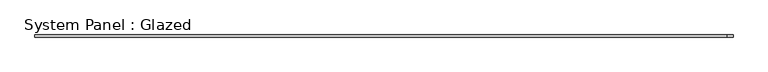
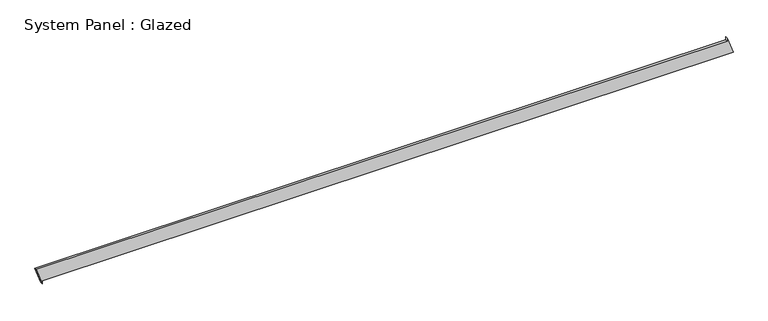
"""IFC4 building model written with IfcOpenShell, lengths in millimetres: plate geometry, System Panel : Glazed."""

import ifcopenshell
import ifcopenshell.guid

model = None  # the IFC model being written
_history = None  # IfcOwnerHistory: only IFC2X3 demands one
_inside = {}  # id of a spatial element -> (the spatial element, [elements in it])
_under = {}  # id of a project, library or spatial element -> (it, [spatial elements below it])
_declared = {}  # id of a project -> (the project, [libraries it declares])
_typed = {}  # id of a type object -> (the type object, [elements of that type])
_made_of = {}  # id of a material, layer set ... -> (it, [elements and type objects made of it])


def new_model(schema):
    """Start an empty IFC model of exactly this schema.

    Asked for "IFC4X3", IfcOpenShell would pick the latest addendum, in which some entities
    have other attributes; the version numbers below select the first issue.
    IFC2X3 requires an IfcOwnerHistory on every rooted entity: one is made here for all.
    """
    global model, _history
    if schema == "IFC4X3":
        model = ifcopenshell.file(schema_version=(4, 3, 0, 0))
    else:
        model = ifcopenshell.file(schema=schema)
    _inside.clear()
    _under.clear()
    _declared.clear()
    _typed.clear()
    _made_of.clear()
    _history = None
    if model.schema == "IFC2X3":
        org = make("IfcOrganization", Name="unknown")
        user = make(
            "IfcPersonAndOrganization",
            ThePerson=make("IfcPerson", FamilyName="unknown"),
            TheOrganization=org,
        )
        app = make(
            "IfcApplication",
            ApplicationDeveloper=org,
            Version="unknown",
            ApplicationFullName="unknown",
            ApplicationIdentifier="unknown",
        )
        _history = make(
            "IfcOwnerHistory",
            OwningUser=user,
            OwningApplication=app,
            ChangeAction="ADDED",
            CreationDate=0,
        )
    return model


def make(cls, **values):
    """One entity of the class cls with the attributes given. An attribute that is None is left unset."""
    return model.create_entity(
        cls, **{name: value for name, value in values.items() if value is not None}
    )


def rooted(cls, **values):
    """An entity with a GlobalId (a new one), such as an element, a storey or a relation."""
    return make(cls, GlobalId=ifcopenshell.guid.new(), OwnerHistory=_history, **values)


def si_unit(unit_type, name, prefix=None):
    """IfcSIUnit, for example si_unit("LENGTHUNIT", "METRE", prefix="MILLI")."""
    return make("IfcSIUnit", UnitType=unit_type, Prefix=prefix, Name=name)


def assignment(units):
    """IfcUnitAssignment: the units of a project."""
    return None if units is None else make("IfcUnitAssignment", Units=units)


def point(xyz):
    """IfcCartesianPoint."""
    return None if xyz is None else make("IfcCartesianPoint", Coordinates=xyz)


def direction(xyz):
    """IfcDirection."""
    return None if xyz is None else make("IfcDirection", DirectionRatios=xyz)


def frame(location, z_axis=None, x_axis=None):
    """IfcAxis2Placement3D, a coordinate frame: its origin and axes. An axis left out is left unset."""
    return make(
        "IfcAxis2Placement3D",
        Location=point(location),
        Axis=direction(z_axis),
        RefDirection=direction(x_axis),
    )


def origin():
    """The frame at (0, 0, 0) with its axes left unset."""
    return frame((0.0, 0.0, 0.0))


def place(relative_to, where):
    """IfcLocalPlacement: puts the frame where relative to a parent placement (None: the world)."""
    return make(
        "IfcLocalPlacement", PlacementRelTo=relative_to, RelativePlacement=where
    )


def context(
    kind, dimensions, precision=None, world=None, true_north=None, identifier=None
):
    """IfcGeometricRepresentationContext, for example the 3D "Model" context."""
    return make(
        "IfcGeometricRepresentationContext",
        ContextIdentifier=identifier,
        ContextType=kind,
        CoordinateSpaceDimension=dimensions,
        Precision=precision,
        WorldCoordinateSystem=world,
        TrueNorth=true_north,
    )


def project(units=None, contexts=None):
    """IfcProject with its units and contexts."""
    return rooted(
        "IfcProject",
        Name="project",
        RepresentationContexts=contexts,
        UnitsInContext=assignment(units),
    )


def spatial(cls, under=None, at=None, **own):
    """A site, building, storey or space (cls), placed at a placement, below another one or the project."""
    s = rooted(cls, ObjectPlacement=at, **own)
    if under is not None:
        _under.setdefault(under.id(), (under, []))[1].append(s)
    return s


def polyline(points):
    """IfcPolyline through the points."""
    return make("IfcPolyline", Points=[point(p) for p in points])


def outline(outer, holes=None, kind="AREA"):
    """IfcArbitraryClosedProfileDef: a profile drawn as a closed curve; with holes, ...WithVoids."""
    if holes is None:
        return make("IfcArbitraryClosedProfileDef", ProfileType=kind, OuterCurve=outer)
    return make(
        "IfcArbitraryProfileDefWithVoids",
        ProfileType=kind,
        OuterCurve=outer,
        InnerCurves=holes,
    )


def extrude(swept, where, along, depth):
    """IfcExtrudedAreaSolid: the profile swept, set in the frame where, extruded along a direction by depth."""
    return make(
        "IfcExtrudedAreaSolid",
        SweptArea=swept,
        Position=where,
        ExtrudedDirection=direction(along),
        Depth=depth,
    )


def shape(context_of_items, identifier, shape_type, items):
    """IfcShapeRepresentation: the items that make up one representation, for example the "Body"."""
    return make(
        "IfcShapeRepresentation",
        ContextOfItems=context_of_items,
        RepresentationIdentifier=identifier,
        RepresentationType=shape_type,
        Items=items,
    )


def source(mapping_origin, context_of_items, identifier, shape_type, items):
    """IfcRepresentationMap: a shape defined once, which mapped items show again and again."""
    return make(
        "IfcRepresentationMap",
        MappingOrigin=mapping_origin,
        MappedRepresentation=shape(context_of_items, identifier, shape_type, items),
    )


def transform(
    local_origin,
    x_axis=None,
    y_axis=None,
    z_axis=None,
    scale=None,
    scale2=None,
    scale3=None,
    uniform=True,
):
    """IfcCartesianTransformationOperator3D, or its non-uniform kind. x_axis, y_axis, z_axis: its Axis1, 2, 3."""
    if uniform:
        return make(
            "IfcCartesianTransformationOperator3D",
            Axis1=direction(x_axis),
            Axis2=direction(y_axis),
            LocalOrigin=point(local_origin),
            Scale=scale,
            Axis3=direction(z_axis),
        )
    return make(
        "IfcCartesianTransformationOperator3DnonUniform",
        Axis1=direction(x_axis),
        Axis2=direction(y_axis),
        LocalOrigin=point(local_origin),
        Scale=scale,
        Axis3=direction(z_axis),
        Scale2=scale2,
        Scale3=scale3,
    )


def mapped(mapping_source, mapping_target):
    """IfcMappedItem: shows the shape of a source again, moved by a transform."""
    return make(
        "IfcMappedItem", MappingSource=mapping_source, MappingTarget=mapping_target
    )


def made_of(thing, what):
    """Note that an element or type object is made of a material, layer set ...; save() writes the relation."""
    if what is not None:
        _made_of.setdefault(what.id(), (what, []))[1].append(thing)
    return thing


def element(
    cls,
    number,
    at=None,
    inside=None,
    cuts=None,
    type_object=None,
    material=None,
    context=None,
    identifier="Body",
    shape_type=None,
    held_by="IfcProductDefinitionShape",
    body=None,
    shapes=None,
    **own,
):
    """One element of the class cls, such as IfcWall. Its Tag is "e" and its number.

    at: its placement. inside: the storey or other place that contains it. cuts: it is an
    opening in that element (IfcRelVoidsElement). A single representation is given by context,
    identifier, shape_type and body (its items); several are given by shapes. held_by: the class
    of the entity that holds the representations. save() writes the other relations.
    """
    e = rooted(cls, Tag="e%d" % number, ObjectPlacement=at, **own)
    if body is not None:
        shapes = [shape(context, identifier, shape_type, body)]
    if shapes is not None:
        e.Representation = make(held_by, Representations=shapes)
    if inside is not None:
        _inside.setdefault(inside.id(), (inside, []))[1].append(e)
    if cuts is not None:
        rooted(
            "IfcRelVoidsElement", RelatingBuildingElement=cuts, RelatedOpeningElement=e
        )
    if type_object is not None:
        _typed.setdefault(type_object.id(), (type_object, []))[1].append(e)
    return made_of(e, material)


def aggregate(whole, parts):
    """IfcRelAggregates: a whole, such as a stair, and the parts it consists of."""
    return rooted("IfcRelAggregates", RelatingObject=whole, RelatedObjects=parts)


def save(model, path):
    """Write the relations noted so far, then the file.

    IfcRelAggregates (storeys below a building ...), IfcRelContainedInSpatialStructure (elements
    in a storey), IfcRelDefinesByType, IfcRelAssociatesMaterial and IfcRelDeclares: one each for
    every whole, place, type object, material and project.
    """
    for whole, parts in _under.values():
        aggregate(whole, parts)
    for where, things in _inside.values():
        rooted(
            "IfcRelContainedInSpatialStructure",
            RelatedElements=things,
            RelatingStructure=where,
        )
    for kind, things in _typed.values():
        rooted("IfcRelDefinesByType", RelatedObjects=things, RelatingType=kind)
    for what, things in _made_of.values():
        rooted("IfcRelAssociatesMaterial", RelatedObjects=things, RelatingMaterial=what)
    for by, libraries in _declared.values():
        rooted("IfcRelDeclares", RelatingContext=by, RelatedDefinitions=libraries)
    model.write(path)


def system_panel_glazed_c66885b6(model_context):
    return source(origin(), model_context, "Body", "SweptSolid", [
        extrude(outline(polyline([(0.0, -3956.9172633), (35.3553391, -3956.9172633), (35.3553391, 4026.9889068), (234.167386, 3956.9192133), (198.8120469, 3956.919217), (198.8112207, -4026.9889068), (0.0, -3956.9172633)])), frame((0.0, -49.5, 0.0), z_axis=(0.0, 1.0, 0.0), x_axis=(0.0, 0.0, 1.0)), (0.0, 0.0, 1.0), 25.0),
    ])


if __name__ == "__main__":
    model = new_model("IFC4")
    model_context = context("Model", 3, world=origin())
    ifc_project = project(units=[si_unit("LENGTHUNIT", "METRE", prefix="MILLI")], contexts=[model_context])
    site = spatial("IfcSite", under=ifc_project)
    building = spatial("IfcBuilding", under=site)
    placement = place(None, origin())
    system_panel_glazed_shape = system_panel_glazed_c66885b6(model_context)
    element("IfcPlate", 1, ObjectType="System Panel : Glazed", at=placement, inside=building, context=model_context, shape_type="MappedRepresentation", body=[
        mapped(system_panel_glazed_shape, transform((0.0, 0.0, 0.0), x_axis=(1.0, 0.0, 0.0), y_axis=(0.0, 1.0, 0.0), z_axis=(0.0, 0.0, 1.0))),
    ])
    save(model, "model.ifc")

# Revit data of these elements
# Element 1 (IfcPlate, "System Panel : Glazed")
#   Materials on its faces: "Glass"
# Materials
#   "Glass": class "Glass", colour RGB 218 227 224, transparency 0.85, Description = "Soda Lime Glass", Cost = 0
